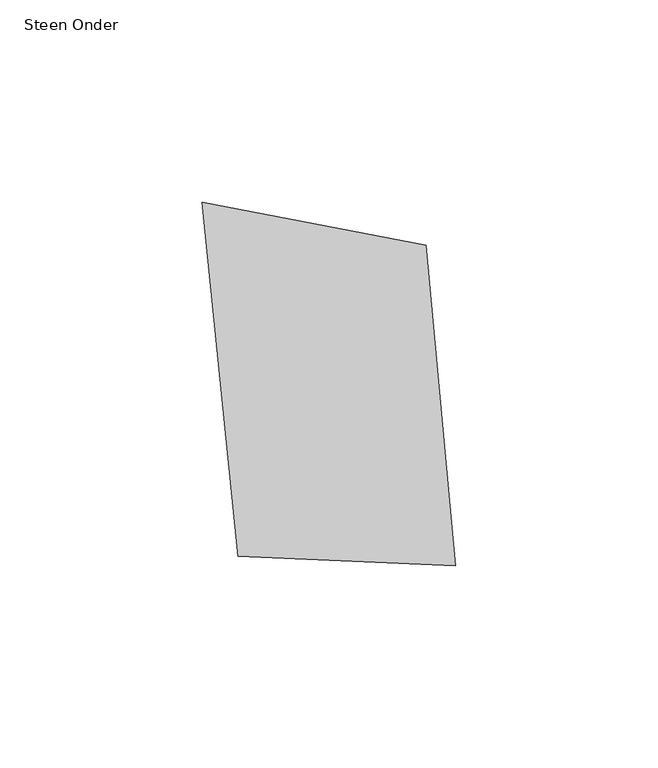
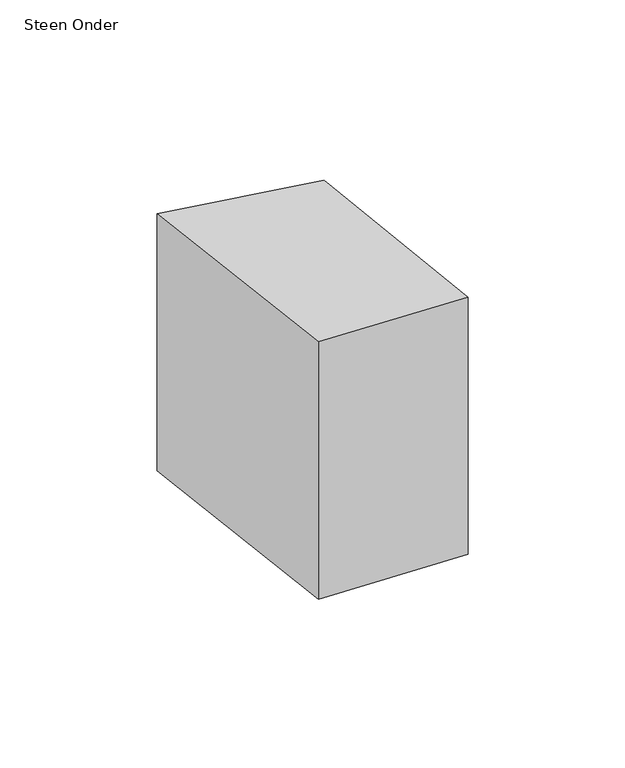
"""IFC4 building model written with IfcOpenShell, lengths in millimetres: proxy geometry, 00_GMA_steen_versie_4 : Steen Onder."""

import ifcopenshell
import ifcopenshell.guid

model = None  # the IFC model being written
_history = None  # IfcOwnerHistory: only IFC2X3 demands one
_inside = {}  # id of a spatial element -> (the spatial element, [elements in it])
_under = {}  # id of a project, library or spatial element -> (it, [spatial elements below it])
_declared = {}  # id of a project -> (the project, [libraries it declares])
_typed = {}  # id of a type object -> (the type object, [elements of that type])
_made_of = {}  # id of a material, layer set ... -> (it, [elements and type objects made of it])


def new_model(schema):
    """Start an empty IFC model of exactly this schema.

    Asked for "IFC4X3", IfcOpenShell would pick the latest addendum, in which some entities
    have other attributes; the version numbers below select the first issue.
    IFC2X3 requires an IfcOwnerHistory on every rooted entity: one is made here for all.
    """
    global model, _history
    if schema == "IFC4X3":
        model = ifcopenshell.file(schema_version=(4, 3, 0, 0))
    else:
        model = ifcopenshell.file(schema=schema)
    _inside.clear()
    _under.clear()
    _declared.clear()
    _typed.clear()
    _made_of.clear()
    _history = None
    if model.schema == "IFC2X3":
        org = make("IfcOrganization", Name="unknown")
        user = make(
            "IfcPersonAndOrganization",
            ThePerson=make("IfcPerson", FamilyName="unknown"),
            TheOrganization=org,
        )
        app = make(
            "IfcApplication",
            ApplicationDeveloper=org,
            Version="unknown",
            ApplicationFullName="unknown",
            ApplicationIdentifier="unknown",
        )
        _history = make(
            "IfcOwnerHistory",
            OwningUser=user,
            OwningApplication=app,
            ChangeAction="ADDED",
            CreationDate=0,
        )
    return model


def make(cls, **values):
    """One entity of the class cls with the attributes given. An attribute that is None is left unset."""
    return model.create_entity(
        cls, **{name: value for name, value in values.items() if value is not None}
    )


def rooted(cls, **values):
    """An entity with a GlobalId (a new one), such as an element, a storey or a relation."""
    return make(cls, GlobalId=ifcopenshell.guid.new(), OwnerHistory=_history, **values)


def si_unit(unit_type, name, prefix=None):
    """IfcSIUnit, for example si_unit("LENGTHUNIT", "METRE", prefix="MILLI")."""
    return make("IfcSIUnit", UnitType=unit_type, Prefix=prefix, Name=name)


def assignment(units):
    """IfcUnitAssignment: the units of a project."""
    return None if units is None else make("IfcUnitAssignment", Units=units)


def point(xyz):
    """IfcCartesianPoint."""
    return None if xyz is None else make("IfcCartesianPoint", Coordinates=xyz)


def direction(xyz):
    """IfcDirection."""
    return None if xyz is None else make("IfcDirection", DirectionRatios=xyz)


def frame(location, z_axis=None, x_axis=None):
    """IfcAxis2Placement3D, a coordinate frame: its origin and axes. An axis left out is left unset."""
    return make(
        "IfcAxis2Placement3D",
        Location=point(location),
        Axis=direction(z_axis),
        RefDirection=direction(x_axis),
    )


def origin():
    """The frame at (0, 0, 0) with its axes left unset."""
    return frame((0.0, 0.0, 0.0))


def origin_with_axes():
    """The frame at (0, 0, 0) with the z axis (0, 0, 1) and the x axis (1, 0, 0) written out."""
    return frame((0.0, 0.0, 0.0), z_axis=(0.0, 0.0, 1.0), x_axis=(1.0, 0.0, 0.0))


def place(relative_to, where):
    """IfcLocalPlacement: puts the frame where relative to a parent placement (None: the world)."""
    return make(
        "IfcLocalPlacement", PlacementRelTo=relative_to, RelativePlacement=where
    )


def context(
    kind, dimensions, precision=None, world=None, true_north=None, identifier=None
):
    """IfcGeometricRepresentationContext, for example the 3D "Model" context."""
    return make(
        "IfcGeometricRepresentationContext",
        ContextIdentifier=identifier,
        ContextType=kind,
        CoordinateSpaceDimension=dimensions,
        Precision=precision,
        WorldCoordinateSystem=world,
        TrueNorth=true_north,
    )


def project(units=None, contexts=None):
    """IfcProject with its units and contexts."""
    return rooted(
        "IfcProject",
        Name="project",
        RepresentationContexts=contexts,
        UnitsInContext=assignment(units),
    )


def spatial(cls, under=None, at=None, **own):
    """A site, building, storey or space (cls), placed at a placement, below another one or the project."""
    s = rooted(cls, ObjectPlacement=at, **own)
    if under is not None:
        _under.setdefault(under.id(), (under, []))[1].append(s)
    return s


def polyline(points):
    """IfcPolyline through the points."""
    return make("IfcPolyline", Points=[point(p) for p in points])


def outline(outer, holes=None, kind="AREA"):
    """IfcArbitraryClosedProfileDef: a profile drawn as a closed curve; with holes, ...WithVoids."""
    if holes is None:
        return make("IfcArbitraryClosedProfileDef", ProfileType=kind, OuterCurve=outer)
    return make(
        "IfcArbitraryProfileDefWithVoids",
        ProfileType=kind,
        OuterCurve=outer,
        InnerCurves=holes,
    )


def extrude(swept, where, along, depth):
    """IfcExtrudedAreaSolid: the profile swept, set in the frame where, extruded along a direction by depth."""
    return make(
        "IfcExtrudedAreaSolid",
        SweptArea=swept,
        Position=where,
        ExtrudedDirection=direction(along),
        Depth=depth,
    )


def shape(context_of_items, identifier, shape_type, items):
    """IfcShapeRepresentation: the items that make up one representation, for example the "Body"."""
    return make(
        "IfcShapeRepresentation",
        ContextOfItems=context_of_items,
        RepresentationIdentifier=identifier,
        RepresentationType=shape_type,
        Items=items,
    )


def source(mapping_origin, context_of_items, identifier, shape_type, items):
    """IfcRepresentationMap: a shape defined once, which mapped items show again and again."""
    return make(
        "IfcRepresentationMap",
        MappingOrigin=mapping_origin,
        MappedRepresentation=shape(context_of_items, identifier, shape_type, items),
    )


def transform(
    local_origin,
    x_axis=None,
    y_axis=None,
    z_axis=None,
    scale=None,
    scale2=None,
    scale3=None,
    uniform=True,
):
    """IfcCartesianTransformationOperator3D, or its non-uniform kind. x_axis, y_axis, z_axis: its Axis1, 2, 3."""
    if uniform:
        return make(
            "IfcCartesianTransformationOperator3D",
            Axis1=direction(x_axis),
            Axis2=direction(y_axis),
            LocalOrigin=point(local_origin),
            Scale=scale,
            Axis3=direction(z_axis),
        )
    return make(
        "IfcCartesianTransformationOperator3DnonUniform",
        Axis1=direction(x_axis),
        Axis2=direction(y_axis),
        LocalOrigin=point(local_origin),
        Scale=scale,
        Axis3=direction(z_axis),
        Scale2=scale2,
        Scale3=scale3,
    )


def mapped(mapping_source, mapping_target):
    """IfcMappedItem: shows the shape of a source again, moved by a transform."""
    return make(
        "IfcMappedItem", MappingSource=mapping_source, MappingTarget=mapping_target
    )


def made_of(thing, what):
    """Note that an element or type object is made of a material, layer set ...; save() writes the relation."""
    if what is not None:
        _made_of.setdefault(what.id(), (what, []))[1].append(thing)
    return thing


def element(
    cls,
    number,
    at=None,
    inside=None,
    cuts=None,
    type_object=None,
    material=None,
    context=None,
    identifier="Body",
    shape_type=None,
    held_by="IfcProductDefinitionShape",
    body=None,
    shapes=None,
    **own,
):
    """One element of the class cls, such as IfcWall. Its Tag is "e" and its number.

    at: its placement. inside: the storey or other place that contains it. cuts: it is an
    opening in that element (IfcRelVoidsElement). A single representation is given by context,
    identifier, shape_type and body (its items); several are given by shapes. held_by: the class
    of the entity that holds the representations. save() writes the other relations.
    """
    e = rooted(cls, Tag="e%d" % number, ObjectPlacement=at, **own)
    if body is not None:
        shapes = [shape(context, identifier, shape_type, body)]
    if shapes is not None:
        e.Representation = make(held_by, Representations=shapes)
    if inside is not None:
        _inside.setdefault(inside.id(), (inside, []))[1].append(e)
    if cuts is not None:
        rooted(
            "IfcRelVoidsElement", RelatingBuildingElement=cuts, RelatedOpeningElement=e
        )
    if type_object is not None:
        _typed.setdefault(type_object.id(), (type_object, []))[1].append(e)
    return made_of(e, material)


def aggregate(whole, parts):
    """IfcRelAggregates: a whole, such as a stair, and the parts it consists of."""
    return rooted("IfcRelAggregates", RelatingObject=whole, RelatedObjects=parts)


def save(model, path):
    """Write the relations noted so far, then the file.

    IfcRelAggregates (storeys below a building ...), IfcRelContainedInSpatialStructure (elements
    in a storey), IfcRelDefinesByType, IfcRelAssociatesMaterial and IfcRelDeclares: one each for
    every whole, place, type object, material and project.
    """
    for whole, parts in _under.values():
        aggregate(whole, parts)
    for where, things in _inside.values():
        rooted(
            "IfcRelContainedInSpatialStructure",
            RelatedElements=things,
            RelatingStructure=where,
        )
    for kind, things in _typed.values():
        rooted("IfcRelDefinesByType", RelatedObjects=things, RelatingType=kind)
    for what, things in _made_of.values():
        rooted("IfcRelAssociatesMaterial", RelatedObjects=things, RelatingMaterial=what)
    for by, libraries in _declared.values():
        rooted("IfcRelDeclares", RelatingContext=by, RelatedDefinitions=libraries)
    model.write(path)


def steen_onder_b195b438(model_context):
    return source(origin(), model_context, "Body", "SweptSolid", [
        extrude(outline(polyline([(97.1753057, 106.4282162), (104.512782, 27.2815183), (50.8262235, 29.5711984), (41.9142715, 116.9802044), (97.1753057, 106.4282162)])), origin_with_axes(), (0.0, 0.0, 1.0), 100.0),
    ])


if __name__ == "__main__":
    model = new_model("IFC4")
    model_context = context("Model", 3, world=origin())
    ifc_project = project(units=[si_unit("LENGTHUNIT", "METRE", prefix="MILLI")], contexts=[model_context])
    site = spatial("IfcSite", under=ifc_project)
    building = spatial("IfcBuilding", under=site)
    placement = place(None, origin())
    steen_onder_shape = steen_onder_b195b438(model_context)
    element("IfcBuildingElementProxy", 1, Name="00_GMA_steen_versie_4 : Steen Onder", ObjectType="00_GMA_steen_versie_4 : Steen Onder", at=placement, inside=building, context=model_context, shape_type="MappedRepresentation", body=[
        mapped(steen_onder_shape, transform((0.0, 0.0, 0.0), x_axis=(1.0, 0.0, 0.0), y_axis=(0.0, 1.0, 0.0), z_axis=(0.0, 0.0, 1.0))),
    ])
    save(model, "model.ifc")

# Revit data of these elements
# Type "00_GMA_steen_versie_4 : Steen Onder"
#   StootVoegHalfBoven [instance default] = 5 mm
#   StootVoegHalf [instance default] = 5 mm
#   StootVoegBreedteOnder = 10 mm
#   StootVoegBreedteBoven = 10 mm
#   Steendikte = 100 mm
#   LintVoegOnderHalf = 0 mm
#   LintVoegOnder = 0 mm
#   LintVoegBovenHalf = 5 mm
#   LintVoegBoven = 10 mm
#   materiaal = none
#   MateriaalVoeg = none
#   Default Elevation = 0
